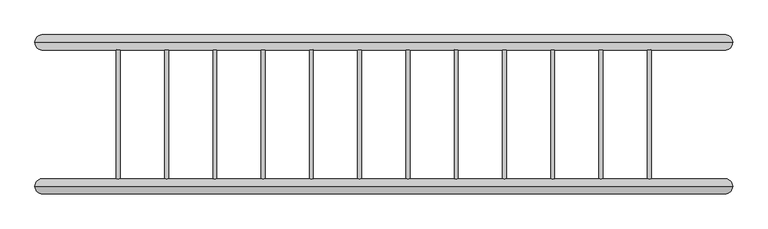
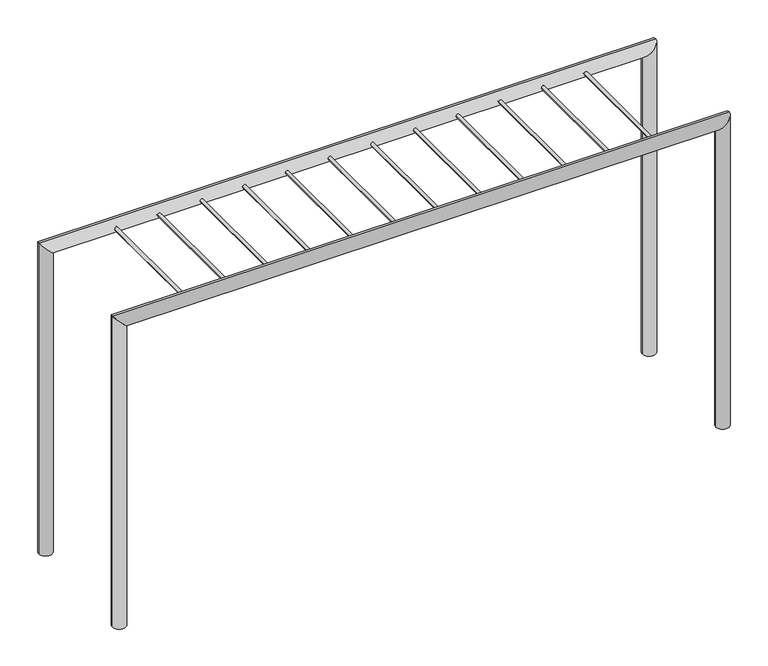
"""IFC4 building model written with IfcOpenShell, lengths in millimetres: proxy geometry, NLRS_90_GM_UN_klimrek_gen_rsf : klimrek 4500x950x2400."""

from ifc_helpers import new_model, si_unit, point, frame, frame_2d, origin, place, context, project, spatial, circle_curve, ellipse_curve, trimmed, segment, composite_curve, outline, extrude, source, transform, mapped, element, save
from ifc_brep_helpers import plane_surface, cylinder_surface, advanced_brep


def generic_models_9b599e35(model_context):
    return source(origin(), model_context, "Body", "SolidModel", [
        extrude(outline(composite_curve([segment(trimmed(circle_curve(frame_2d((2400.0, 1431.8181818)), 12.7), [point((2400.0, 1419.1181818))], [point((2400.0, 1444.5181818))], False, "CARTESIAN"), True, "CONTINUOUS"), segment(trimmed(circle_curve(frame_2d((2400.0, 1431.8181818)), 12.7), [point((2400.0, 1444.5181818))], [point((2400.0, 1419.1181818))], False, "CARTESIAN"), True, "CONTINUOUS")], self_intersect=False)), frame((0.0, -475.0, 0.0), z_axis=(0.0, 1.0, 0.0), x_axis=(0.0, 0.0, 1.0)), (0.0, 0.0, 1.0), 950.0),
        extrude(outline(composite_curve([segment(trimmed(circle_curve(frame_2d((2400.0, 1113.6363636)), 12.7), [point((2400.0, 1100.9363636))], [point((2400.0, 1126.3363636))], False, "CARTESIAN"), True, "CONTINUOUS"), segment(trimmed(circle_curve(frame_2d((2400.0, 1113.6363636)), 12.7), [point((2400.0, 1126.3363636))], [point((2400.0, 1100.9363636))], False, "CARTESIAN"), True, "CONTINUOUS")], self_intersect=False)), frame((0.0, -475.0, 0.0), z_axis=(0.0, 1.0, 0.0), x_axis=(0.0, 0.0, 1.0)), (0.0, 0.0, 1.0), 950.0),
        extrude(outline(composite_curve([segment(trimmed(circle_curve(frame_2d((2400.0, 795.4545455)), 12.7), [point((2400.0, 782.7545455))], [point((2400.0, 808.1545455))], False, "CARTESIAN"), True, "CONTINUOUS"), segment(trimmed(circle_curve(frame_2d((2400.0, 795.4545455)), 12.7), [point((2400.0, 808.1545455))], [point((2400.0, 782.7545455))], False, "CARTESIAN"), True, "CONTINUOUS")], self_intersect=False)), frame((0.0, -475.0, 0.0), z_axis=(0.0, 1.0, 0.0), x_axis=(0.0, 0.0, 1.0)), (0.0, 0.0, 1.0), 950.0),
        extrude(outline(composite_curve([segment(trimmed(circle_curve(frame_2d((2400.0, 477.2727273)), 12.7), [point((2400.0, 464.5727273))], [point((2400.0, 489.9727273))], False, "CARTESIAN"), True, "CONTINUOUS"), segment(trimmed(circle_curve(frame_2d((2400.0, 477.2727273)), 12.7), [point((2400.0, 489.9727273))], [point((2400.0, 464.5727273))], False, "CARTESIAN"), True, "CONTINUOUS")], self_intersect=False)), frame((0.0, -475.0, 0.0), z_axis=(0.0, 1.0, 0.0), x_axis=(0.0, 0.0, 1.0)), (0.0, 0.0, 1.0), 950.0),
        extrude(outline(composite_curve([segment(trimmed(circle_curve(frame_2d((2400.0, 159.0909091)), 12.7), [point((2400.0, 146.3909091))], [point((2400.0, 171.7909091))], False, "CARTESIAN"), True, "CONTINUOUS"), segment(trimmed(circle_curve(frame_2d((2400.0, 159.0909091)), 12.7), [point((2400.0, 171.7909091))], [point((2400.0, 146.3909091))], False, "CARTESIAN"), True, "CONTINUOUS")], self_intersect=False)), frame((0.0, -475.0, 0.0), z_axis=(0.0, 1.0, 0.0), x_axis=(0.0, 0.0, 1.0)), (0.0, 0.0, 1.0), 950.0),
        extrude(outline(composite_curve([segment(trimmed(circle_curve(frame_2d((2400.0, -159.0909091)), 12.7), [point((2400.0, -171.7909091))], [point((2400.0, -146.3909091))], False, "CARTESIAN"), True, "CONTINUOUS"), segment(trimmed(circle_curve(frame_2d((2400.0, -159.0909091)), 12.7), [point((2400.0, -146.3909091))], [point((2400.0, -171.7909091))], False, "CARTESIAN"), True, "CONTINUOUS")], self_intersect=False)), frame((0.0, -475.0, 0.0), z_axis=(0.0, 1.0, 0.0), x_axis=(0.0, 0.0, 1.0)), (0.0, 0.0, 1.0), 950.0),
        extrude(outline(composite_curve([segment(trimmed(circle_curve(frame_2d((2400.0, -477.2727273)), 12.7), [point((2400.0, -489.9727273))], [point((2400.0, -464.5727273))], False, "CARTESIAN"), True, "CONTINUOUS"), segment(trimmed(circle_curve(frame_2d((2400.0, -477.2727273)), 12.7), [point((2400.0, -464.5727273))], [point((2400.0, -489.9727273))], False, "CARTESIAN"), True, "CONTINUOUS")], self_intersect=False)), frame((0.0, -475.0, 0.0), z_axis=(0.0, 1.0, 0.0), x_axis=(0.0, 0.0, 1.0)), (0.0, 0.0, 1.0), 950.0),
        extrude(outline(composite_curve([segment(trimmed(circle_curve(frame_2d((2400.0, -795.4545455)), 12.7), [point((2400.0, -808.1545455))], [point((2400.0, -782.7545455))], False, "CARTESIAN"), True, "CONTINUOUS"), segment(trimmed(circle_curve(frame_2d((2400.0, -795.4545455)), 12.7), [point((2400.0, -782.7545455))], [point((2400.0, -808.1545455))], False, "CARTESIAN"), True, "CONTINUOUS")], self_intersect=False)), frame((0.0, -475.0, 0.0), z_axis=(0.0, 1.0, 0.0), x_axis=(0.0, 0.0, 1.0)), (0.0, 0.0, 1.0), 950.0),
        extrude(outline(composite_curve([segment(trimmed(circle_curve(frame_2d((2400.0, -1113.6363636)), 12.7), [point((2400.0, -1126.3363636))], [point((2400.0, -1100.9363636))], False, "CARTESIAN"), True, "CONTINUOUS"), segment(trimmed(circle_curve(frame_2d((2400.0, -1113.6363636)), 12.7), [point((2400.0, -1100.9363636))], [point((2400.0, -1126.3363636))], False, "CARTESIAN"), True, "CONTINUOUS")], self_intersect=False)), frame((0.0, -475.0, 0.0), z_axis=(0.0, 1.0, 0.0), x_axis=(0.0, 0.0, 1.0)), (0.0, 0.0, 1.0), 950.0),
        extrude(outline(composite_curve([segment(trimmed(circle_curve(frame_2d((2400.0, -1431.8181818)), 12.7), [point((2400.0, -1444.5181818))], [point((2400.0, -1419.1181818))], False, "CARTESIAN"), True, "CONTINUOUS"), segment(trimmed(circle_curve(frame_2d((2400.0, -1431.8181818)), 12.7), [point((2400.0, -1419.1181818))], [point((2400.0, -1444.5181818))], False, "CARTESIAN"), True, "CONTINUOUS")], self_intersect=False)), frame((0.0, -475.0, 0.0), z_axis=(0.0, 1.0, 0.0), x_axis=(0.0, 0.0, 1.0)), (0.0, 0.0, 1.0), 950.0),
        extrude(outline(composite_curve([segment(trimmed(circle_curve(frame_2d((2400.0, 1750.0)), 12.7), [point((2400.0, 1737.3))], [point((2400.0, 1762.7))], False, "CARTESIAN"), True, "CONTINUOUS"), segment(trimmed(circle_curve(frame_2d((2400.0, 1750.0)), 12.7), [point((2400.0, 1762.7))], [point((2400.0, 1737.3))], False, "CARTESIAN"), True, "CONTINUOUS")], self_intersect=False)), frame((0.0, -475.0, 0.0), z_axis=(0.0, 1.0, 0.0), x_axis=(0.0, 0.0, 1.0)), (0.0, 0.0, 1.0), 950.0),
        extrude(outline(composite_curve([segment(trimmed(circle_curve(frame_2d((2400.0, -1750.0)), 12.7), [point((2400.0, -1762.7))], [point((2400.0, -1737.3))], False, "CARTESIAN"), True, "CONTINUOUS"), segment(trimmed(circle_curve(frame_2d((2400.0, -1750.0)), 12.7), [point((2400.0, -1737.3))], [point((2400.0, -1762.7))], False, "CARTESIAN"), True, "CONTINUOUS")], self_intersect=False)), frame((0.0, -475.0, 0.0), z_axis=(0.0, 1.0, 0.0), x_axis=(0.0, 0.0, 1.0)), (0.0, 0.0, 1.0), 950.0),
        advanced_brep(
        [(-2200.0, -475.0, 0.0), (-2300.0, -475.0, 0.0), (-2300.0, -475.0, 2450.0), (-2200.0, -475.0, 2350.0), (2200.0, -475.0, 0.0), (2300.0, -475.0, 0.0), (2200.0, -475.0, 2350.0), (2300.0, -475.0, 2450.0)],
        [
            (0, 1, circle_curve(frame((-2250.0, -475.0, 0.0), z_axis=(0.0, 0.0, -1.0), x_axis=(-1.0, 0.0, 0.0)), 50.0)),
            (1, 0, circle_curve(frame((-2250.0, -475.0, 0.0), z_axis=(0.0, 0.0, -1.0), x_axis=(-1.0, 0.0, 0.0)), 50.0)),
            (1, 2),
            (2, 3, ellipse_curve(frame((-2250.0, -475.0, 2400.0), z_axis=(-0.7071067811865475, 0.0, -0.7071067811865475), x_axis=(0.7071067811865474, 0.0, -0.7071067811865476)), 70.7106781, 50.0)),
            (3, 0),
            (3, 2, ellipse_curve(frame((-2250.0, -475.0, 2400.0), z_axis=(-0.7071067811865475, 0.0, -0.7071067811865475), x_axis=(0.7071067811865474, 0.0, -0.7071067811865476)), 70.7106781, 50.0)),
            (4, 5, circle_curve(frame((2250.0, -475.0, 0.0), z_axis=(0.0, 0.0, -1.0), x_axis=(1.0, 0.0, 0.0)), 50.0)),
            (5, 4, circle_curve(frame((2250.0, -475.0, 0.0), z_axis=(0.0, 0.0, -1.0), x_axis=(1.0, 0.0, 0.0)), 50.0)),
            (6, 4),
            (5, 7),
            (7, 6, ellipse_curve(frame((2250.0, -475.0, 2400.0), z_axis=(0.7071067811865475, 0.0, -0.7071067811865475), x_axis=(0.7071067811865474, 0.0, 0.7071067811865476)), 70.7106781, 50.0)),
            (6, 7, ellipse_curve(frame((2250.0, -475.0, 2400.0), z_axis=(0.7071067811865475, 0.0, -0.7071067811865475), x_axis=(0.7071067811865474, 0.0, 0.7071067811865476)), 70.7106781, 50.0)),
            (2, 7),
            (6, 3),
        ],
        [
            plane_surface(frame((-2250.0, -475.0, 0.0), z_axis=(0.0, 0.0, -1.0), x_axis=(0.0, 1.0, 0.0))),
            cylinder_surface(frame((-2250.0, -475.0, 0.0), z_axis=(0.0, 0.0, -1.0), x_axis=(-1.0, 0.0, 0.0)), 50.0),
            plane_surface(frame((2250.0, -475.0, 0.0), z_axis=(0.0, 0.0, -1.0), x_axis=(0.0, 1.0, 0.0))),
            cylinder_surface(frame((2250.0, -475.0, 2400.0), z_axis=(0.0, 0.0, 1.0), x_axis=(1.0, 0.0, 0.0)), 50.0),
            cylinder_surface(frame((-2250.0, -475.0, 2400.0), z_axis=(-1.0, 0.0, 0.0), x_axis=(0.0, 0.0, 1.0)), 50.0),
        ],
        [
            (0, [[1, 2]]),
            (1, [[3, 4, 5, -2]]),
            (1, [[-5, 6, -3, -1]]),
            (2, [[7, 8]]),
            (3, [[9, -8, 10, 11]]),
            (3, [[-10, -7, -9, 12]]),
            (4, [[13, -12, 14, -4]]),
            (4, [[-14, -11, -13, -6]]),
        ],
    ),
        advanced_brep(
        [(2200.0, 475.0, 0.0), (2300.0, 475.0, 0.0), (2200.0, 475.0, 2350.0), (2300.0, 475.0, 2450.0), (-2200.0, 475.0, 2350.0), (-2300.0, 475.0, 2450.0), (-2200.0, 475.0, 0.0), (-2300.0, 475.0, 0.0)],
        [
            (0, 1, circle_curve(frame((2250.0, 475.0, 0.0), z_axis=(0.0, 0.0, -1.0), x_axis=(1.0, 0.0, 0.0)), 50.0)),
            (1, 0, circle_curve(frame((2250.0, 475.0, 0.0), z_axis=(0.0, 0.0, -1.0), x_axis=(1.0, 0.0, 0.0)), 50.0)),
            (0, 2),
            (2, 3, ellipse_curve(frame((2250.0, 475.0, 2400.0), z_axis=(0.7071067811865475, 0.0, -0.7071067811865475), x_axis=(-0.7071067811865474, 0.0, -0.7071067811865476)), 70.7106781, 50.0)),
            (3, 1),
            (3, 2, ellipse_curve(frame((2250.0, 475.0, 2400.0), z_axis=(0.7071067811865475, 0.0, -0.7071067811865475), x_axis=(-0.7071067811865474, 0.0, -0.7071067811865476)), 70.7106781, 50.0)),
            (2, 4),
            (4, 5, ellipse_curve(frame((-2250.0, 475.0, 2400.0), z_axis=(0.7071067811865475, 0.0, 0.7071067811865475), x_axis=(0.7071067811865476, 0.0, -0.7071067811865474)), 70.7106781, 50.0)),
            (5, 3),
            (5, 4, ellipse_curve(frame((-2250.0, 475.0, 2400.0), z_axis=(0.7071067811865475, 0.0, 0.7071067811865475), x_axis=(0.7071067811865476, 0.0, -0.7071067811865474)), 70.7106781, 50.0)),
            (6, 7, circle_curve(frame((-2250.0, 475.0, 0.0), z_axis=(0.0, 0.0, -1.0), x_axis=(-1.0, 0.0, 0.0)), 50.0)),
            (7, 6, circle_curve(frame((-2250.0, 475.0, 0.0), z_axis=(0.0, 0.0, -1.0), x_axis=(-1.0, 0.0, 0.0)), 50.0)),
            (4, 6),
            (7, 5),
        ],
        [
            plane_surface(frame((2250.0, 475.0, 0.0), z_axis=(0.0, 0.0, -1.0), x_axis=(0.0, 1.0, 0.0))),
            cylinder_surface(frame((2250.0, 475.0, 0.0), z_axis=(0.0, 0.0, -1.0), x_axis=(1.0, 0.0, 0.0)), 50.0),
            cylinder_surface(frame((2250.0, 475.0, 2400.0), z_axis=(1.0, 0.0, 0.0), x_axis=(0.0, 0.0, 1.0)), 50.0),
            plane_surface(frame((-2250.0, 475.0, 0.0), z_axis=(0.0, 0.0, -1.0), x_axis=(0.0, 1.0, 0.0))),
            cylinder_surface(frame((-2250.0, 475.0, 2400.0), z_axis=(0.0, 0.0, 1.0), x_axis=(-1.0, 0.0, 0.0)), 50.0),
        ],
        [
            (0, [[1, 2]]),
            (1, [[-1, 3, 4, 5]]),
            (1, [[-2, -5, 6, -3]]),
            (2, [[-4, 7, 8, 9]]),
            (2, [[-6, -9, 10, -7]]),
            (3, [[11, 12]]),
            (4, [[-8, 13, -12, 14]]),
            (4, [[-10, -14, -11, -13]]),
        ],
    ),
    ])


if __name__ == "__main__":
    model = new_model("IFC4")
    model_context = context("Model", 3, world=origin())
    ifc_project = project(units=[si_unit("LENGTHUNIT", "METRE", prefix="MILLI")], contexts=[model_context])
    site = spatial("IfcSite", under=ifc_project)
    building = spatial("IfcBuilding", under=site)
    placement = place(None, origin())
    generic_models_shape = generic_models_9b599e35(model_context)
    element("IfcBuildingElementProxy", 1, Name="NLRS_90_GM_UN_klimrek_gen_rsf : klimrek 4500x950x2400", ObjectType="NLRS_90_GM_UN_klimrek_gen_rsf : klimrek 4500x950x2400", at=placement, inside=building, context=model_context, shape_type="MappedRepresentation", body=[
        mapped(generic_models_shape, transform((0.0, 0.0, 0.0), x_axis=(1.0, 0.0, 0.0), y_axis=(0.0, 1.0, 0.0), z_axis=(0.0, 0.0, 1.0))),
    ])
    save(model, "model.ifc")

# Revit data of these elements
# Type "NLRS_90_GM_UN_klimrek_gen_rsf : klimrek 4500x950x2400"
#   Type IFC Predefined Type = "USERDEFINED"
#   Export Type to IFC As = "IfcGeographicElementType"
#   Type IfcGUID = "05J6pyYiTDtR2exmlhyPk6"
#   IfcName[Type] = "klimrek 4500x950x2400"
#   IfcDescription[Type] = "klimrek lxbxh 4500x950x2400mm"
#   IfcObjectType[Type] = "PLAYGROUND"
#   IfcExportAs[Type] = "IfcGeographicElementType"
#   IfcExportType[Type] = "USERDEFINED"
#   NLRS_C_revit_versie = ""
#   NLRS_C_omschrijving_02 [instance default] = "sporten"
#   NLRS_C_omschrijving_01 [instance default] = "frame"
#   NLRS_C_content_versie = ""
#   NLRS_C_content_provider = ""
#   NLRS_C_content_handleiding = ""
#   NLRS_C_content_datum_uitgifte = ""
#   NLRS_C_content_datum_gewijzigd = ""
#   NLRS_C_content_creator = ""
#   Model = "generiek"
#   Manufacturer = "Revit Standards Foundation"
#   Description = "klimrek lxbxh 4500x950x2400mm"
#   Assembly Code = "90.71"
#   NLRS_C_lengte_02 = 3500.00 mm
#   NLRS_C_lengte = 4500.00 mm
#   NLRS_C_hoogte = 2400.00 mm
#   NLRS_C_breedte = 950.00 mm
#   NLRS_C_aantal_02 = 12
#   NLRS_C_materiaal_02 = NLRS_h_metaal wit_gen_rsf
#   NLRS_C_materiaal_01 = NLRS_a_generiek materiaal rood-RGB213-27-23_gen_rsf
#   Default Elevation = 0
# Element 1 (IfcBuildingElementProxy, "NLRS_90_GM_UN_klimrek_gen_rsf : klimrek 4500x950x2400")
#   Materials on its faces: "NLRS_h_metaal wit_gen_rsf", "NLRS_a_generiek materiaal rood-RGB213-27-23_gen_rsf"
# Materials
#   "NLRS_h_metaal wit_gen_rsf": class "Metal", colour RGB 237 237 237, transparency 0, Keynote = "h", Model = "generiek", Manufacturer = "Revit Standards Foundation", URL = "www.revitstandards.org", Description = "metaal wit", Cost = 0
#   "NLRS_a_generiek materiaal rood-RGB213-27-23_gen_rsf": class "Metal", colour RGB 213 27 23, transparency 0, Keynote = "a", Model = "generiek", Manufacturer = "Revit Standards Foundation", URL = "www.revitstandards.org", Description = "kleur rood", Cost = 0
